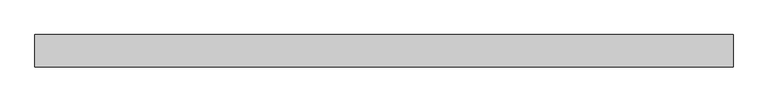
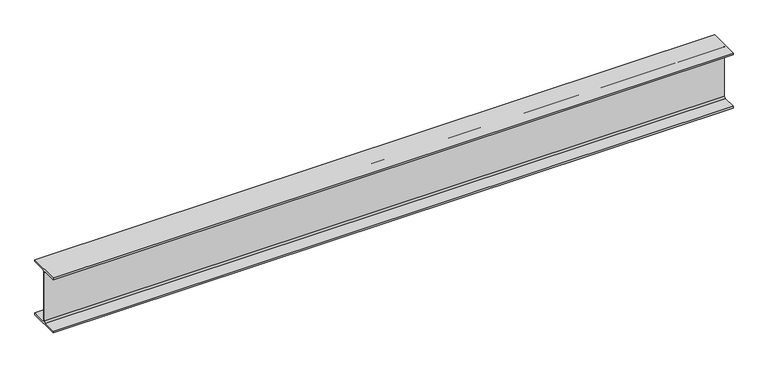
"""IFC4 building model written with IfcOpenShell, lengths in millimetres: beam geometry, Old_Steel Beam_H-KSD3502 : H_SB_ASB_H-200×200x8x12."""

from ifc_helpers import new_model, si_unit, point, frame, frame_2d, origin, place, context, project, spatial, polyline, circle_curve, trimmed, segment, composite_curve, outline, extrude, source, transform, mapped, element, save


def beam_7328ca8b(model_context):
    return source(origin(), model_context, "Body", "SweptSolid", [
        extrude(outline(composite_curve([segment(polyline([(82.5, -141.5), (82.5, -151.7), (-82.5, -151.7), (-82.5, -141.5), (-11.9, -141.5)]), True, "CONTINUOUS"), segment(trimmed(circle_curve(frame_2d((-11.9, -132.6)), 8.9), [point((-11.9, -141.5))], [point((-3.0, -132.6))], True, "CARTESIAN"), True, "CONTINUOUS"), segment(polyline([(-3.0, -132.6), (-3.0, 132.6)]), True, "CONTINUOUS"), segment(trimmed(circle_curve(frame_2d((-11.9, 132.6)), 8.9), [point((-3.0, 132.6))], [point((-11.9, 141.5))], True, "CARTESIAN"), True, "CONTINUOUS"), segment(polyline([(-11.9, 141.5), (-82.5, 141.5), (-82.5, 151.7), (82.5, 151.7), (82.5, 141.5), (11.9, 141.5)]), True, "CONTINUOUS"), segment(trimmed(circle_curve(frame_2d((11.9, 132.6)), 8.9), [point((11.9, 141.5))], [point((3.0, 132.6))], True, "CARTESIAN"), True, "CONTINUOUS"), segment(polyline([(3.0, 132.6), (3.0, -132.6)]), True, "CONTINUOUS"), segment(trimmed(circle_curve(frame_2d((11.9, -132.6)), 8.9), [point((3.0, -132.6))], [point((11.9, -141.5))], True, "CARTESIAN"), True, "CONTINUOUS"), segment(polyline([(11.9, -141.5), (82.5, -141.5)]), True, "CONTINUOUS")], self_intersect=False)), frame((-1725.502423, 0.0, 0.0), z_axis=(1.0, 0.0, 0.0), x_axis=(0.0, 1.0, 0.0)), (0.0, 0.0, 1.0), 3536.3433078),
    ])


if __name__ == "__main__":
    model = new_model("IFC4")
    model_context = context("Model", 3, world=origin())
    ifc_project = project(units=[si_unit("LENGTHUNIT", "METRE", prefix="MILLI")], contexts=[model_context])
    site = spatial("IfcSite", under=ifc_project)
    building = spatial("IfcBuilding", under=site)
    placement = place(None, origin())
    beam_shape = beam_7328ca8b(model_context)
    element("IfcBeam", 1, ObjectType="Old_Steel Beam_H-KSD3502 : H_SB_ASB_H-200×200x8x12", at=placement, inside=building, context=model_context, shape_type="MappedRepresentation", body=[
        mapped(beam_shape, transform((0.0, 0.0, 0.0), x_axis=(1.0, 0.0, 0.0), y_axis=(0.0, 1.0, 0.0), z_axis=(0.0, 0.0, 1.0))),
    ])
    save(model, "model.ifc")

# Revit data of these elements
# Type "Old_Steel Beam_H-KSD3502 : H_SB_ASB_H-200×200x8x12"
#   Width = 20.0 cm
#   Web Thickness = 0.8 cm
#   Web Fillet = 1.3 cm
#   Warping Constant = 141376.0 cm⁶
#   Torsional Moment of Inertia = 26.2485 cm⁴
#   Torsional Modulus = 1.0 cm³
#   Section Area = 63.53 cm²
#   Plastic Modulus weak axis = 244.0 cm³
#   Plastic Modulus strong axis = 525.0 cm³
#   Perimeter = 1.16 m²/m
#   Nominal Weight = 49.90 kgf/m
#   Moment of Inertia weak axis = 1600.00 cm⁴
#   Moment of Inertia strong axis = 4720.00 cm⁴
#   Height = 20.0 cm
#   Flange Thickness = 1.2 cm
#   Elastic Modulus weak axis = 160.0 cm³
#   Elastic Modulus strong axis = 472.0 cm³
#   Centroid Vertical = 10.0 cm
#   Centroid Horizontal = 10.0 cm
#   Length [instance default] = 1.5240 m
#   Structural Material [instance default] = Steel, 45-345
#   Assembly Code = ""
# Element 1 (IfcBeam, "Old_Steel Beam_H-KSD3502 : H_SB_ASB_H-200×200x8x12")
#   Structural Material = none
# Materials
#   "Steel, 45-345": class "Metal", colour RGB 189 187 185, transparency 0, Description = "Steel 345 MPa", Cost = 0
